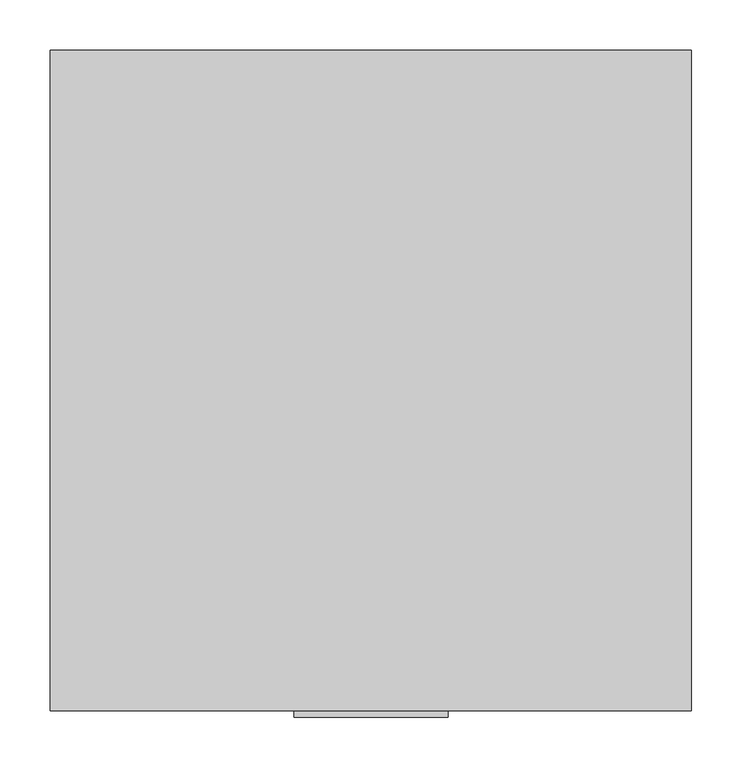
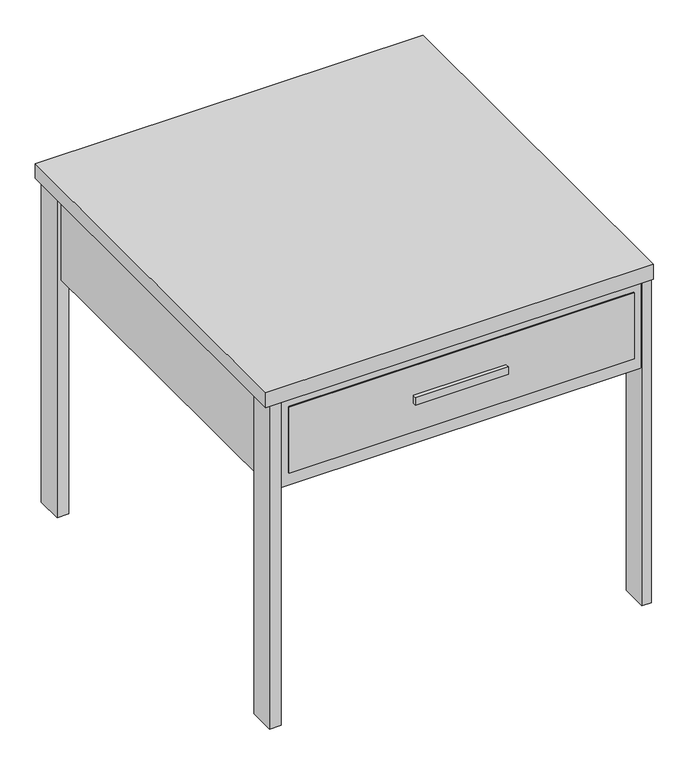
"""IFC4 building model written with IfcOpenShell, lengths in millimetres: furniture geometry, End Table-NON-COLLECTUS : -."""

from ifc_helpers import new_model, si_unit, frame, origin, origin_with_axes, place, context, project, spatial, polyline, outline, extrude, source, transform, mapped, element, save


def furniture_c15940ef(model_context):
    return source(origin(), model_context, "Body", "SweptSolid", [
        extrude(outline(polyline([(76.2, -660.4), (-76.2, -660.4), (-76.2, -654.05), (76.2, -654.05), (76.2, -660.4)])), frame((0.0, 0.0, 482.6), z_axis=(0.0, 0.0, 1.0), x_axis=(1.0, 0.0, 0.0)), (0.0, 0.0, 1.0), 12.7),
        extrude(outline(polyline([(285.75, -654.05), (-279.4, -654.05), (-279.4, -609.6), (285.75, -609.6), (285.75, -654.05)])), frame((0.0, 0.0, 431.8), z_axis=(0.0, 0.0, 1.0), x_axis=(1.0, 0.0, 0.0)), (0.0, 0.0, 1.0), 114.3),
        extrude(outline(polyline([(304.8, -6.35), (304.8, -652.1648438), (-304.8, -652.1648438), (-304.8, -6.35), (304.8, -6.35)])), frame((0.0, 0.0, 410.0734835), z_axis=(0.0, 0.0, 1.0), x_axis=(1.0, 0.0, 0.0)), (0.0, 0.0, 1.0), 148.7265165),
        extrude(outline(polyline([(317.5, 0.0), (317.5, -654.05), (-317.5, -654.05), (-317.5, 0.0), (317.5, 0.0)])), frame((0.0, 0.0, 558.8), z_axis=(0.0, 0.0, 1.0), x_axis=(1.0, 0.0, 0.0)), (0.0, 0.0, 1.0), 25.4),
        extrude(outline(polyline([(-292.1, -6.35), (-292.1, -50.8), (-311.15, -50.8), (-311.15, -6.35), (-292.1, -6.35)])), origin_with_axes(), (0.0, 0.0, 1.0), 558.8),
        extrude(outline(polyline([(314.2881053, -6.35), (314.2881053, -50.8), (298.45, -50.8), (298.45, -6.35), (314.2881053, -6.35)])), origin_with_axes(), (0.0, 0.0, 1.0), 558.8),
        extrude(outline(polyline([(314.2881053, -609.6), (314.2881053, -654.05), (298.45, -654.05), (298.45, -609.6), (314.2881053, -609.6)])), origin_with_axes(), (0.0, 0.0, 1.0), 558.8),
        extrude(outline(polyline([(-292.1, -609.6), (-292.1, -654.05), (-311.15, -654.05), (-311.15, -609.6), (-292.1, -609.6)])), origin_with_axes(), (0.0, 0.0, 1.0), 558.8),
    ])


if __name__ == "__main__":
    model = new_model("IFC4")
    model_context = context("Model", 3, world=origin())
    ifc_project = project(units=[si_unit("LENGTHUNIT", "METRE", prefix="MILLI")], contexts=[model_context])
    site = spatial("IfcSite", under=ifc_project)
    building = spatial("IfcBuilding", under=site)
    placement = place(None, origin())
    furniture_shape = furniture_c15940ef(model_context)
    element("IfcFurniture", 1, ObjectType="End Table-NON-COLLECTUS : -", at=placement, inside=building, context=model_context, shape_type="MappedRepresentation", body=[
        mapped(furniture_shape, transform((0.0, 0.0, 0.0), x_axis=(1.0, 0.0, 0.0), y_axis=(0.0, 1.0, 0.0), z_axis=(0.0, 0.0, 1.0))),
    ])
    save(model, "model.ifc")

# Revit data of these elements
# Type "End Table-NON-COLLECTUS : -"
#   External ID [instance default] = ""
#   Width = 635 mm
#   Height = 584.2 mm
#   Depth = 660.4 mm
#   Drawer [instance default] = yes
#   Material = White
#   Default Elevation = 0
# Element 1 (IfcFurniture, "End Table-NON-COLLECTUS : -")
#   Materials on its faces: "White"
# Materials
#   "White": class "Generic", colour RGB 255 255 255, transparency 0, Cost = 0
